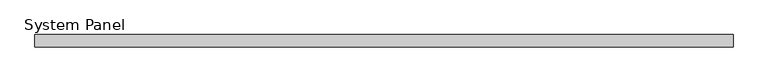
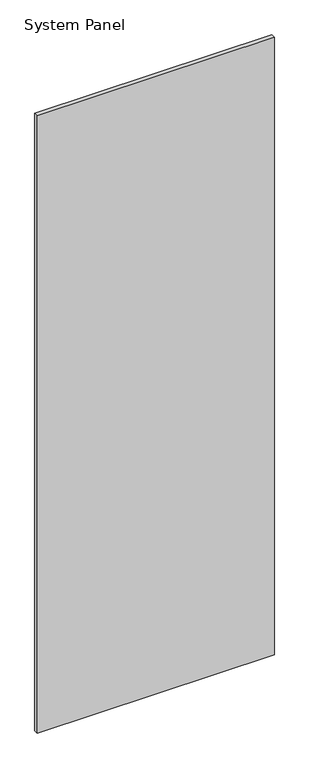
"""IFC4 building model written with IfcOpenShell, lengths in millimetres: plate geometry, System Panel : WWm-Glass-20mm-10mmOffset."""

from ifc_helpers import new_model, si_unit, origin, origin_with_axes, place, context, project, spatial, polyline, outline, extrude, source, transform, mapped, element, save


def system_panel_b13e0cf2(model_context):
    return source(origin(), model_context, "Body", "SweptSolid", [
        extrude(outline(polyline([(572.6771401, 0.0), (-572.6771401, 0.0), (-572.6771401, 20.0), (572.6771401, 20.0), (572.6771401, 0.0)])), origin_with_axes(), (0.0, 0.0, 1.0), 3150.0),
    ])


if __name__ == "__main__":
    model = new_model("IFC4")
    model_context = context("Model", 3, world=origin())
    ifc_project = project(units=[si_unit("LENGTHUNIT", "METRE", prefix="MILLI")], contexts=[model_context])
    site = spatial("IfcSite", under=ifc_project)
    building = spatial("IfcBuilding", under=site)
    placement = place(None, origin())
    system_panel_shape = system_panel_b13e0cf2(model_context)
    element("IfcPlate", 1, ObjectType="System Panel : WWm-Glass-20mm-10mmOffset", at=placement, inside=building, context=model_context, shape_type="MappedRepresentation", body=[
        mapped(system_panel_shape, transform((0.0, 0.0, 0.0), x_axis=(1.0, 0.0, 0.0), y_axis=(0.0, 1.0, 0.0), z_axis=(0.0, 0.0, 1.0))),
    ])
    save(model, "model.ifc")

# Revit data of these elements
# Type "System Panel : WWm-Glass-20mm-10mmOffset"
#   Finish = ""
# Element 1 (IfcPlate, "System Panel : WWm-Glass-20mm-10mmOffset")
#   Materials on its faces: "WW-EC-GL-Storefront"
# Materials
#   "WW-EC-GL-Storefront": class "Glass", colour RGB 236 240 239, transparency 0.85, Description = "Storefront Glass", Cost = 0
